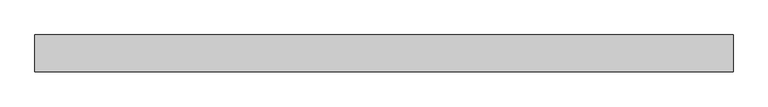
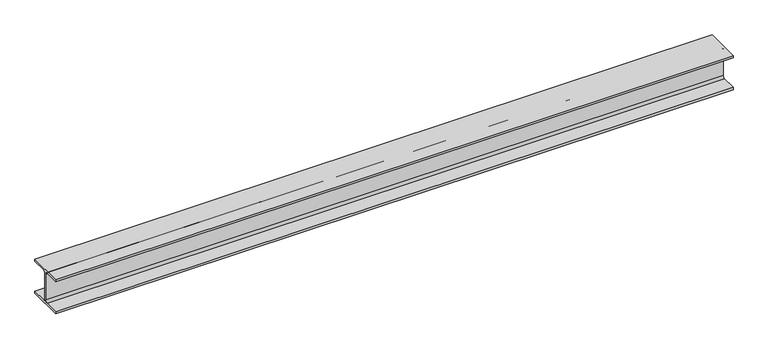
"""IFC4 building model written with IfcOpenShell, lengths in millimetres: beam geometry, 0912_Steel Framing_H-KSD3502 : H_SB_ASB_H-200x200x8x12."""

from ifc_helpers import new_model, si_unit, point, frame, frame_2d, origin, place, context, project, spatial, polyline, circle_curve, trimmed, segment, composite_curve, outline, extrude, source, transform, mapped, element, save


def beam_d0f8d902(model_context):
    return source(origin(), model_context, "Body", "SweptSolid", [
        extrude(outline(composite_curve([segment(polyline([(100.0, -88.0), (100.0, -100.0), (-100.0, -100.0), (-100.0, -88.0), (-17.0, -88.0)]), True, "CONTINUOUS"), segment(trimmed(circle_curve(frame_2d((-17.0, -75.0)), 13.0), [point((-17.0, -88.0))], [point((-4.0, -75.0))], True, "CARTESIAN"), True, "CONTINUOUS"), segment(polyline([(-4.0, -75.0), (-4.0, 75.0)]), True, "CONTINUOUS"), segment(trimmed(circle_curve(frame_2d((-17.0, 75.0)), 13.0), [point((-4.0, 75.0))], [point((-17.0, 88.0))], True, "CARTESIAN"), True, "CONTINUOUS"), segment(polyline([(-17.0, 88.0), (-100.0, 88.0), (-100.0, 100.0), (100.0, 100.0), (100.0, 88.0), (17.0, 88.0)]), True, "CONTINUOUS"), segment(trimmed(circle_curve(frame_2d((17.0, 75.0)), 13.0), [point((17.0, 88.0))], [point((4.0, 75.0))], True, "CARTESIAN"), True, "CONTINUOUS"), segment(polyline([(4.0, 75.0), (4.0, -75.0)]), True, "CONTINUOUS"), segment(trimmed(circle_curve(frame_2d((17.0, -75.0)), 13.0), [point((4.0, -75.0))], [point((17.0, -88.0))], True, "CARTESIAN"), True, "CONTINUOUS"), segment(polyline([(17.0, -88.0), (100.0, -88.0)]), True, "CONTINUOUS")], self_intersect=False)), frame((-1944.4205415, 0.0, 0.0), z_axis=(1.0, 0.0, 0.0), x_axis=(0.0, 1.0, 0.0)), (0.0, 0.0, 1.0), 3769.1418816),
    ])


if __name__ == "__main__":
    model = new_model("IFC4")
    model_context = context("Model", 3, world=origin())
    ifc_project = project(units=[si_unit("LENGTHUNIT", "METRE", prefix="MILLI")], contexts=[model_context])
    site = spatial("IfcSite", under=ifc_project)
    building = spatial("IfcBuilding", under=site)
    placement = place(None, origin())
    beam_shape = beam_d0f8d902(model_context)
    element("IfcBeam", 1, ObjectType="0912_Steel Framing_H-KSD3502 : H_SB_ASB_H-200x200x8x12", at=placement, inside=building, context=model_context, shape_type="MappedRepresentation", body=[
        mapped(beam_shape, transform((0.0, 0.0, 0.0), x_axis=(1.0, 0.0, 0.0), y_axis=(0.0, 1.0, 0.0), z_axis=(0.0, 0.0, 1.0))),
    ])
    save(model, "model.ifc")

# Revit data of these elements
# Type "0912_Steel Framing_H-KSD3502 : H_SB_ASB_H-200x200x8x12"
#   H_WM Code_1 = "S01AA002-00001 | Main Steel Structure Fabrication Work | Shelter/Building | Medium Steel - Standard (90KG/M>Weight≥30KG/M) | Material: (   )"
#   H_WM Code_2 = "S03AA028-00001 | Main Steel Structure Erection Work | Shelter/Building | Medium Steel (90KG/M>Weight≥30KG/M) | Material: (   )"
#   H_WM Code_3 = "S01AA010-00001 | Main Steel Structure Fabrication Work | Shelter/Building | Steel Painting/Coating | for Non-Fireproofed Steel Surface, Surface Preparation, Primer, Second & Final Coat | Material: (   )"
#   H_Q'ty Cal Type Tag = "SB-Q2"
#   Width = 20.0 cm
#   Web Thickness = 0.8 cm
#   Web Fillet = 1.3 cm
#   Warping Constant = 141000.0 cm⁶
#   W = 0
#   Torsional Moment of Inertia = 26.2485 cm⁴
#   Section Area = 63.53 cm²
#   Plastic Modulus weak axis = 244.0 cm³
#   Plastic Modulus strong axis = 525.0 cm³
#   Perimeter = 1.16 m²/m
#   Nominal Weight = 49.90 kgf/m
#   Moment of Inertia weak axis = 1600.00 cm⁴
#   Moment of Inertia strong axis = 4720.00 cm⁴
#   Height = 20.0 cm
#   Flange Thickness = 1.2 cm
#   Elastic Modulus weak axis = 160.0 cm³
#   Elastic Modulus strong axis = 472.0 cm³
#   Centroid Vertical = 10.0 cm
#   Centroid Horizontal = 10.0 cm
#   Ix = 47200000
#   Length [instance default] = 1.5240 m
#   Zx = 525000
#   b = 0.2000 m
#   h = 0.2000 m
#   r = 0.0130 m
#   s = 0.0080 m
#   t = 0.0120 m
#   A = 0.006353 m²
#   Structural Material [instance default] = Steel, 45-345
#   Assembly Code = ""
# Element 1 (IfcBeam, "0912_Steel Framing_H-KSD3502 : H_SB_ASB_H-200x200x8x12")
#   Structural Material = none
# Materials
#   "Steel, 45-345": class "Metal", colour RGB 189 187 185, transparency 0, Description = "Steel 345 MPa", Cost = 0
